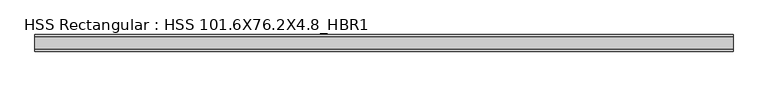
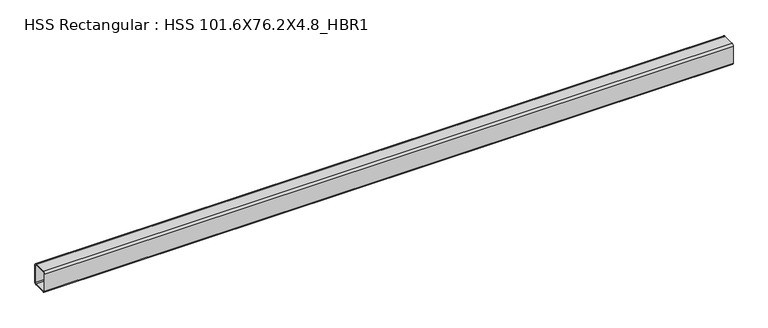
"""IFC4 building model written with IfcOpenShell, lengths in millimetres: beam geometry, HSS Rectangular : HSS 101.6X76.2X4.8_HBR1."""

from ifc_helpers import new_model, si_unit, point, frame, frame_2d, origin, place, context, project, spatial, polyline, circle_curve, trimmed, segment, composite_curve, outline, extrude, source, transform, mapped, element, save


def hss_rectangular_hss_101_6x76_2x4_8_hbr1_0838e563(model_context):
    return source(origin(), model_context, "Body", "SweptSolid", [
        extrude(outline(composite_curve([segment(polyline([(38.1, 41.275), (38.1, -41.275)]), True, "CONTINUOUS"), segment(trimmed(circle_curve(frame_2d((28.575, -41.275)), 9.525), [point((38.1, -41.275))], [point((28.575, -50.8))], False, "CARTESIAN"), True, "CONTINUOUS"), segment(polyline([(28.575, -50.8), (-28.575, -50.8)]), True, "CONTINUOUS"), segment(trimmed(circle_curve(frame_2d((-28.575, -41.275)), 9.525), [point((-28.575, -50.8))], [point((-38.1, -41.275))], False, "CARTESIAN"), True, "CONTINUOUS"), segment(polyline([(-38.1, -41.275), (-38.1, 41.275)]), True, "CONTINUOUS"), segment(trimmed(circle_curve(frame_2d((-28.575, 41.275)), 9.525), [point((-38.1, 41.275))], [point((-28.575, 50.8))], False, "CARTESIAN"), True, "CONTINUOUS"), segment(polyline([(-28.575, 50.8), (28.575, 50.8)]), True, "CONTINUOUS"), segment(trimmed(circle_curve(frame_2d((28.575, 41.275)), 9.525), [point((28.575, 50.8))], [point((38.1, 41.275))], False, "CARTESIAN"), True, "CONTINUOUS")], self_intersect=False), holes=[composite_curve([segment(trimmed(circle_curve(frame_2d((-28.575, 41.275)), 4.7625), [point((-28.575, 46.0375))], [point((-33.3375, 41.275))], True, "CARTESIAN"), True, "CONTINUOUS"), segment(polyline([(-33.3375, 41.275), (-33.3375, -41.275)]), True, "CONTINUOUS"), segment(trimmed(circle_curve(frame_2d((-28.575, -41.275)), 4.7625), [point((-33.3375, -41.275))], [point((-28.575, -46.0375))], True, "CARTESIAN"), True, "CONTINUOUS"), segment(polyline([(-28.575, -46.0375), (28.575, -46.0375)]), True, "CONTINUOUS"), segment(trimmed(circle_curve(frame_2d((28.575, -41.275)), 4.7625), [point((28.575, -46.0375))], [point((33.3375, -41.275))], True, "CARTESIAN"), True, "CONTINUOUS"), segment(polyline([(33.3375, -41.275), (33.3375, 41.275)]), True, "CONTINUOUS"), segment(trimmed(circle_curve(frame_2d((28.575, 41.275)), 4.7625), [point((33.3375, 41.275))], [point((28.575, 46.0375))], True, "CARTESIAN"), True, "CONTINUOUS"), segment(polyline([(28.575, 46.0375), (-28.575, 46.0375)]), True, "CONTINUOUS")], self_intersect=False)]), frame((-1565.6850321, 0.0, 0.0), z_axis=(1.0, 0.0, 0.0), x_axis=(0.0, 1.0, 0.0)), (0.0, 0.0, 1.0), 3204.5027933),
    ])


if __name__ == "__main__":
    model = new_model("IFC4")
    model_context = context("Model", 3, world=origin())
    ifc_project = project(units=[si_unit("LENGTHUNIT", "METRE", prefix="MILLI")], contexts=[model_context])
    site = spatial("IfcSite", under=ifc_project)
    building = spatial("IfcBuilding", under=site)
    placement = place(None, origin())
    hss_rectangular_hss_101_6x76_2x4_8_hbr1_shape = hss_rectangular_hss_101_6x76_2x4_8_hbr1_0838e563(model_context)
    element("IfcBeam", 1, ObjectType="HSS Rectangular : HSS 101.6X76.2X4.8_HBR1", at=placement, inside=building, context=model_context, shape_type="MappedRepresentation", body=[
        mapped(hss_rectangular_hss_101_6x76_2x4_8_hbr1_shape, transform((0.0, 0.0, 0.0), x_axis=(1.0, 0.0, 0.0), y_axis=(0.0, 1.0, 0.0), z_axis=(0.0, 0.0, 1.0))),
    ])
    save(model, "model.ifc")

# Revit data of these elements
# Type "HSS Rectangular : HSS 101.6X76.2X4.8_HBR1"
#   Section Name Key = "HSS 4X3X3/16"
#   Assembly Code = "B10"
#   Width = 7.62 cm
#   Wall Nominal Thickness = 0.4763 cm
#   Wall Design Thickness = 0.442 cm
#   Torsional Moment of Inertia = 260.561 cm⁴
#   Torsional Modulus = 61.2876 cm³
#   Section Area = 14.4516 cm²
#   Plastic Modulus weak axis = 40.3122 cm³
#   Plastic Modulus strong axis = 49.1612 cm³
#   Perimeter = 0.881482 m²/m
#   Outer Fillet = 0.9525 cm
#   Nominal Weight = 12.1285 kgf/m
#   Moment of Inertia weak axis = 131.529 cm⁴
#   Moment of Inertia strong axis = 205.202 cm⁴
#   Inner Fillet = 0.4763 cm
#   Height = 10.16 cm
#   Elastic Modulus weak axis = 34.4128 cm³
#   Elastic Modulus strong axis = 40.476 cm³
#   Centroid Vertical = 5.08 cm
#   Centroid Horizontal = 3.81 cm
#   Length [instance default] = 1524 mm
#   Structural Material [instance default] = Steel ASTM A500, Grade B, Rectangular and Square
#   Principal Axes Angle = 0
# Element 1 (IfcBeam, "HSS Rectangular : HSS 101.6X76.2X4.8_HBR1")
#   Structural Material = Steel ASTM A992
#   Materials on its faces: "Steel ASTM A992"
# Materials
#   "Steel ASTM A500, Grade B, Rectangular and Square": class "Metal", colour RGB 199 199 199, transparency 0, Description = "Carbon steel", Cost = 0
#   "Steel ASTM A992": class "Metal", colour RGB 199 199 199, transparency 0, Description = "Structural steel 50ksi", Cost = 0
